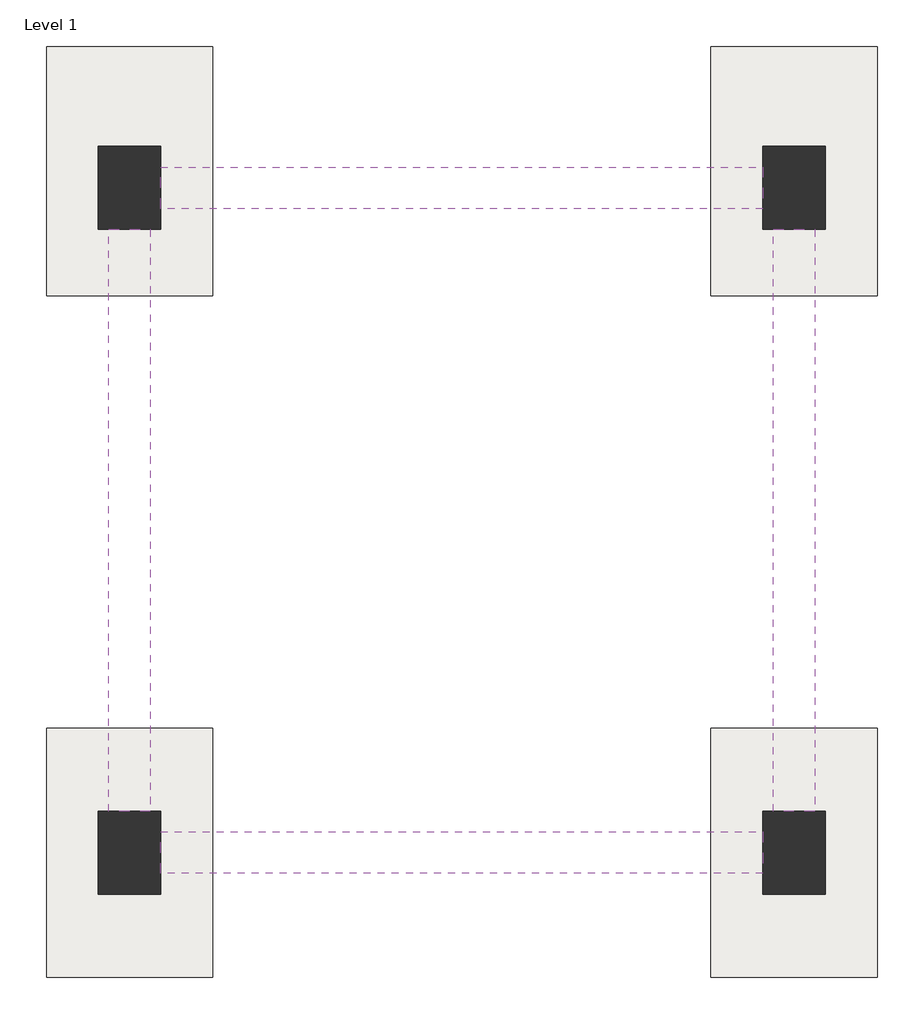
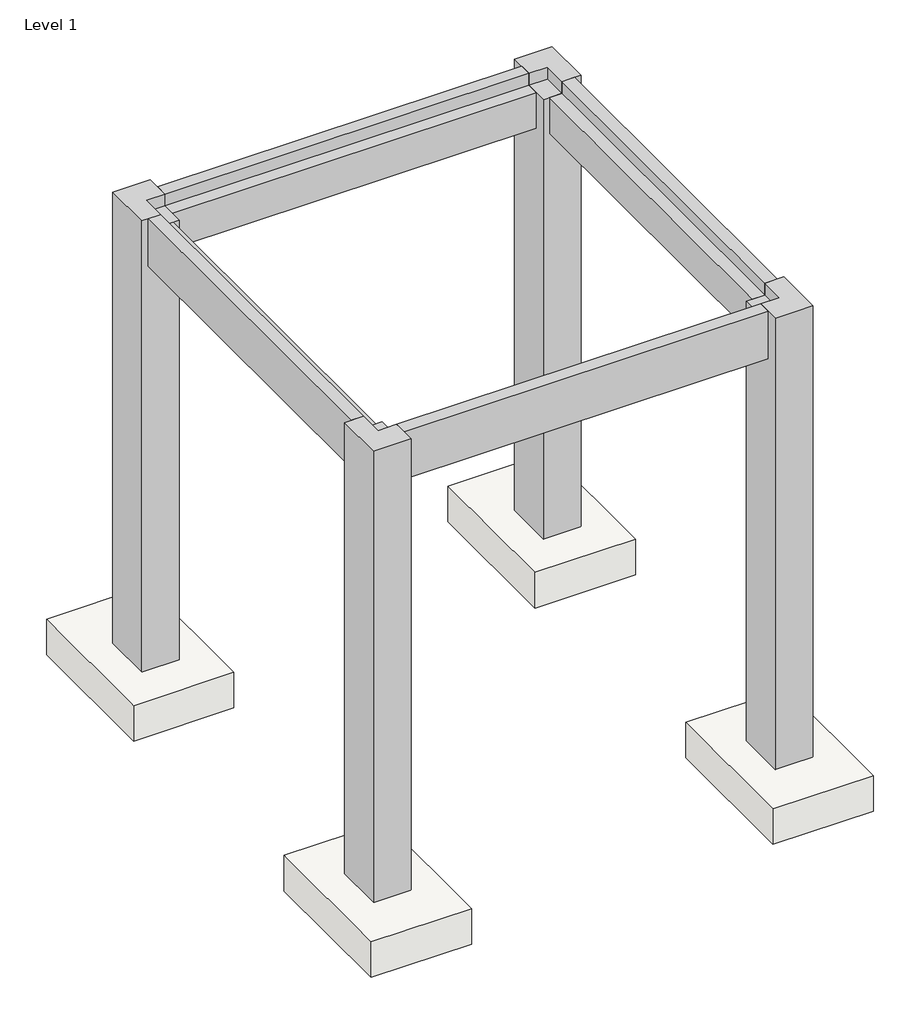
# One storey: 4 beams, 4 columns, 4 slabs.
"""IFC4 building model written with IfcOpenShell, lengths in millimetres."""

import ifcopenshell
import ifcopenshell.guid

model = None  # the IFC model being written
_history = None  # IfcOwnerHistory: only IFC2X3 demands one
_inside = {}  # id of a spatial element -> (the spatial element, [elements in it])
_under = {}  # id of a project, library or spatial element -> (it, [spatial elements below it])
_declared = {}  # id of a project -> (the project, [libraries it declares])
_typed = {}  # id of a type object -> (the type object, [elements of that type])
_made_of = {}  # id of a material, layer set ... -> (it, [elements and type objects made of it])


def new_model(schema):
    """Start an empty IFC model of exactly this schema.

    Asked for "IFC4X3", IfcOpenShell would pick the latest addendum, in which some entities
    have other attributes; the version numbers below select the first issue.
    IFC2X3 requires an IfcOwnerHistory on every rooted entity: one is made here for all.
    """
    global model, _history
    if schema == "IFC4X3":
        model = ifcopenshell.file(schema_version=(4, 3, 0, 0))
    else:
        model = ifcopenshell.file(schema=schema)
    _inside.clear()
    _under.clear()
    _declared.clear()
    _typed.clear()
    _made_of.clear()
    _history = None
    if model.schema == "IFC2X3":
        org = make("IfcOrganization", Name="unknown")
        user = make(
            "IfcPersonAndOrganization",
            ThePerson=make("IfcPerson", FamilyName="unknown"),
            TheOrganization=org,
        )
        app = make(
            "IfcApplication",
            ApplicationDeveloper=org,
            Version="unknown",
            ApplicationFullName="unknown",
            ApplicationIdentifier="unknown",
        )
        _history = make(
            "IfcOwnerHistory",
            OwningUser=user,
            OwningApplication=app,
            ChangeAction="ADDED",
            CreationDate=0,
        )
    return model


def make(cls, **values):
    """One entity of the class cls with the attributes given. An attribute that is None is left unset."""
    return model.create_entity(
        cls, **{name: value for name, value in values.items() if value is not None}
    )


def rooted(cls, **values):
    """An entity with a GlobalId (a new one), such as an element, a storey or a relation."""
    return make(cls, GlobalId=ifcopenshell.guid.new(), OwnerHistory=_history, **values)


def si_unit(unit_type, name, prefix=None):
    """IfcSIUnit, for example si_unit("LENGTHUNIT", "METRE", prefix="MILLI")."""
    return make("IfcSIUnit", UnitType=unit_type, Prefix=prefix, Name=name)


def assignment(units):
    """IfcUnitAssignment: the units of a project."""
    return None if units is None else make("IfcUnitAssignment", Units=units)


def point(xyz):
    """IfcCartesianPoint."""
    return None if xyz is None else make("IfcCartesianPoint", Coordinates=xyz)


def direction(xyz):
    """IfcDirection."""
    return None if xyz is None else make("IfcDirection", DirectionRatios=xyz)


def frame(location, z_axis=None, x_axis=None):
    """IfcAxis2Placement3D, a coordinate frame: its origin and axes. An axis left out is left unset."""
    return make(
        "IfcAxis2Placement3D",
        Location=point(location),
        Axis=direction(z_axis),
        RefDirection=direction(x_axis),
    )


def origin():
    """The frame at (0, 0, 0) with its axes left unset."""
    return frame((0.0, 0.0, 0.0))


def place(relative_to, where):
    """IfcLocalPlacement: puts the frame where relative to a parent placement (None: the world)."""
    return make(
        "IfcLocalPlacement", PlacementRelTo=relative_to, RelativePlacement=where
    )


def context(
    kind, dimensions, precision=None, world=None, true_north=None, identifier=None
):
    """IfcGeometricRepresentationContext, for example the 3D "Model" context."""
    return make(
        "IfcGeometricRepresentationContext",
        ContextIdentifier=identifier,
        ContextType=kind,
        CoordinateSpaceDimension=dimensions,
        Precision=precision,
        WorldCoordinateSystem=world,
        TrueNorth=true_north,
    )


def project(units=None, contexts=None):
    """IfcProject with its units and contexts."""
    return rooted(
        "IfcProject",
        Name="project",
        RepresentationContexts=contexts,
        UnitsInContext=assignment(units),
    )


def spatial(cls, under=None, at=None, **own):
    """A site, building, storey or space (cls), placed at a placement, below another one or the project."""
    s = rooted(cls, ObjectPlacement=at, **own)
    if under is not None:
        _under.setdefault(under.id(), (under, []))[1].append(s)
    return s


def polyline(points):
    """IfcPolyline through the points."""
    return make("IfcPolyline", Points=[point(p) for p in points])


def outline(outer, holes=None, kind="AREA"):
    """IfcArbitraryClosedProfileDef: a profile drawn as a closed curve; with holes, ...WithVoids."""
    if holes is None:
        return make("IfcArbitraryClosedProfileDef", ProfileType=kind, OuterCurve=outer)
    return make(
        "IfcArbitraryProfileDefWithVoids",
        ProfileType=kind,
        OuterCurve=outer,
        InnerCurves=holes,
    )


def extrude(swept, where, along, depth):
    """IfcExtrudedAreaSolid: the profile swept, set in the frame where, extruded along a direction by depth."""
    return make(
        "IfcExtrudedAreaSolid",
        SweptArea=swept,
        Position=where,
        ExtrudedDirection=direction(along),
        Depth=depth,
    )


def faces_of(points, faces, orient=None, outer=None):
    """IfcFace entities. A face is a list of loops; a loop is a list of indices into points, from 0.

    orient and outer hold one flag for each loop. By default every Orientation is true, the
    first loop of a face is its IfcFaceOuterBound and the others are IfcFaceBound.
    """
    made = []
    for i, loops in enumerate(faces):
        bounds = []
        for j, loop in enumerate(loops):
            is_outer = j == 0 if outer is None else outer[i][j]
            bounds.append(
                make(
                    "IfcFaceOuterBound" if is_outer else "IfcFaceBound",
                    Bound=make("IfcPolyLoop", Polygon=[points[k] for k in loop]),
                    Orientation=True if orient is None else orient[i][j],
                )
            )
        made.append(make("IfcFace", Bounds=bounds))
    return made


def faceted_brep(points, faces, orient=None, outer=None, voids=None):
    """IfcFacetedBrep: a solid bounded by flat faces; with voids (closed shells), ...WithVoids."""
    shared = [point(p) for p in points]
    hull = make("IfcClosedShell", CfsFaces=faces_of(shared, faces, orient, outer))
    if voids is None:
        return make("IfcFacetedBrep", Outer=hull)
    return make(
        "IfcFacetedBrepWithVoids",
        Outer=hull,
        Voids=[
            make(cls, CfsFaces=faces_of(shared, fs, o, b)) for cls, fs, o, b in voids
        ],
    )


def shape(context_of_items, identifier, shape_type, items):
    """IfcShapeRepresentation: the items that make up one representation, for example the "Body"."""
    return make(
        "IfcShapeRepresentation",
        ContextOfItems=context_of_items,
        RepresentationIdentifier=identifier,
        RepresentationType=shape_type,
        Items=items,
    )


def source(mapping_origin, context_of_items, identifier, shape_type, items):
    """IfcRepresentationMap: a shape defined once, which mapped items show again and again."""
    return make(
        "IfcRepresentationMap",
        MappingOrigin=mapping_origin,
        MappedRepresentation=shape(context_of_items, identifier, shape_type, items),
    )


def transform(
    local_origin,
    x_axis=None,
    y_axis=None,
    z_axis=None,
    scale=None,
    scale2=None,
    scale3=None,
    uniform=True,
):
    """IfcCartesianTransformationOperator3D, or its non-uniform kind. x_axis, y_axis, z_axis: its Axis1, 2, 3."""
    if uniform:
        return make(
            "IfcCartesianTransformationOperator3D",
            Axis1=direction(x_axis),
            Axis2=direction(y_axis),
            LocalOrigin=point(local_origin),
            Scale=scale,
            Axis3=direction(z_axis),
        )
    return make(
        "IfcCartesianTransformationOperator3DnonUniform",
        Axis1=direction(x_axis),
        Axis2=direction(y_axis),
        LocalOrigin=point(local_origin),
        Scale=scale,
        Axis3=direction(z_axis),
        Scale2=scale2,
        Scale3=scale3,
    )


def mapped(mapping_source, mapping_target):
    """IfcMappedItem: shows the shape of a source again, moved by a transform."""
    return make(
        "IfcMappedItem", MappingSource=mapping_source, MappingTarget=mapping_target
    )


def made_of(thing, what):
    """Note that an element or type object is made of a material, layer set ...; save() writes the relation."""
    if what is not None:
        _made_of.setdefault(what.id(), (what, []))[1].append(thing)
    return thing


def element(
    cls,
    number,
    at=None,
    inside=None,
    cuts=None,
    type_object=None,
    material=None,
    context=None,
    identifier="Body",
    shape_type=None,
    held_by="IfcProductDefinitionShape",
    body=None,
    shapes=None,
    **own,
):
    """One element of the class cls, such as IfcWall. Its Tag is "e" and its number.

    at: its placement. inside: the storey or other place that contains it. cuts: it is an
    opening in that element (IfcRelVoidsElement). A single representation is given by context,
    identifier, shape_type and body (its items); several are given by shapes. held_by: the class
    of the entity that holds the representations. save() writes the other relations.
    """
    e = rooted(cls, Tag="e%d" % number, ObjectPlacement=at, **own)
    if body is not None:
        shapes = [shape(context, identifier, shape_type, body)]
    if shapes is not None:
        e.Representation = make(held_by, Representations=shapes)
    if inside is not None:
        _inside.setdefault(inside.id(), (inside, []))[1].append(e)
    if cuts is not None:
        rooted(
            "IfcRelVoidsElement", RelatingBuildingElement=cuts, RelatedOpeningElement=e
        )
    if type_object is not None:
        _typed.setdefault(type_object.id(), (type_object, []))[1].append(e)
    return made_of(e, material)


def aggregate(whole, parts):
    """IfcRelAggregates: a whole, such as a stair, and the parts it consists of."""
    return rooted("IfcRelAggregates", RelatingObject=whole, RelatedObjects=parts)


def save(model, path):
    """Write the relations noted so far, then the file.

    IfcRelAggregates (storeys below a building ...), IfcRelContainedInSpatialStructure (elements
    in a storey), IfcRelDefinesByType, IfcRelAssociatesMaterial and IfcRelDeclares: one each for
    every whole, place, type object, material and project.
    """
    for whole, parts in _under.values():
        aggregate(whole, parts)
    for where, things in _inside.values():
        rooted(
            "IfcRelContainedInSpatialStructure",
            RelatedElements=things,
            RelatingStructure=where,
        )
    for kind, things in _typed.values():
        rooted("IfcRelDefinesByType", RelatedObjects=things, RelatingType=kind)
    for what, things in _made_of.values():
        rooted("IfcRelAssociatesMaterial", RelatedObjects=things, RelatingMaterial=what)
    for by, libraries in _declared.values():
        rooted("IfcRelDeclares", RelatingContext=by, RelatedDefinitions=libraries)
    model.write(path)


def slab_5ba74754(model_context):
    return source(origin(), model_context, "Body", "SweptSolid", [
        extrude(outline(polyline([(609.6, 914.4), (609.6, -914.4), (-609.6, -914.4), (-609.6, 914.4), (609.6, 914.4)])), frame((0.0, 0.0, -457.2), z_axis=(0.0, 0.0, 1.0), x_axis=(1.0, 0.0, 0.0)), (0.0, 0.0, 1.0), 457.2),
    ])


model = new_model("IFC4")

# Units and contexts
model_context = context("Model", 3, world=origin())
ifc_project = project(units=[si_unit("LENGTHUNIT", "METRE", prefix="MILLI")], contexts=[model_context])

# Site, building, storey
site = spatial("IfcSite", under=ifc_project)
building = spatial("IfcBuilding", under=site)
storey = spatial("IfcBuildingStorey", under=building, Name="Level 1", Elevation=0.0)

# Beams
placement = place(None, origin())
element("IfcBeam", 1, ObjectType="Concrete-Rectangular Beam : 12 x 24", at=placement, inside=storey, context=model_context, shape_type="SweptSolid", body=[
    extrude(outline(polyline([(786.0323826, 2438.4), (786.0323826, 3048.0), (938.4323826, 3048.0), (938.4323826, 2895.6), (1090.8323826, 2895.6), (1090.8323826, 2438.4), (786.0323826, 2438.4)])), frame((-11045.0800525, 0.0, 0.0), z_axis=(1.0, 0.0, 0.0), x_axis=(0.0, 1.0, 0.0)), (0.0, 0.0, 1.0), 4419.6),
])
element("IfcBeam", 2, ObjectType="Concrete-Rectangular Beam : 12 x 24", at=placement, inside=storey, context=model_context, shape_type="SweptSolid", body=[
    extrude(outline(polyline([(5967.6323826, 3048.0), (5967.6323826, 2438.4), (5662.8323826, 2438.4), (5662.8323826, 2895.6), (5815.2323826, 2895.6), (5815.2323826, 3048.0), (5967.6323826, 3048.0)])), frame((-11045.0800525, 0.0, 0.0), z_axis=(1.0, 0.0, 0.0), x_axis=(0.0, 1.0, 0.0)), (0.0, 0.0, 1.0), 4419.6),
])
element("IfcBeam", 3, ObjectType="Concrete-Rectangular Beam : 12 x 24", at=placement, inside=storey, context=model_context, shape_type="SweptSolid", body=[
    extrude(outline(polyline([(2438.4, -11426.0800525), (2438.4, -11121.2800525), (2895.6, -11121.2800525), (2895.6, -11273.6800525), (3048.0, -11273.6800525), (3048.0, -11426.0800525), (2438.4, -11426.0800525)])), frame((0.0, 1243.2323826, 0.0), z_axis=(0.0, 1.0, 0.0), x_axis=(0.0, 0.0, 1.0)), (0.0, 0.0, 1.0), 4267.2),
])
element("IfcBeam", 4, ObjectType="Concrete-Rectangular Beam : 12 x 24", at=placement, inside=storey, context=model_context, shape_type="SweptSolid", body=[
    extrude(outline(polyline([(2438.4, -6244.4800525), (3048.0, -6244.4800525), (3048.0, -6396.8800525), (2895.6, -6396.8800525), (2895.6, -6549.2800525), (2438.4, -6549.2800525), (2438.4, -6244.4800525)])), frame((0.0, 1243.2323826, 0.0), z_axis=(0.0, 1.0, 0.0), x_axis=(0.0, 0.0, 1.0)), (0.0, 0.0, 1.0), 4267.2),
])

# Columns
element("IfcColumn", 5, ObjectType="Concrete-Rectangular-Column : 18 x 24", at=placement, inside=storey, context=model_context, shape_type="Brep", body=[
    faceted_brep([(-11045.0800525, 6120.0323826, 3048.0), (-11502.2800525, 6120.0323826, 3048.0), (-11502.2800525, 5510.4323826, 3048.0), (-11273.6800525, 5510.4323826, 3048.0), (-11273.6800525, 5815.2323826, 3048.0), (-11045.0800525, 5815.2323826, 3048.0), (-11045.0800525, 6120.0323826, -2743.2), (-11045.0800525, 5510.4323826, -2743.2), (-11502.2800525, 5510.4323826, -2743.2), (-11502.2800525, 6120.0323826, -2743.2), (-11045.0800525, 5510.4323826, 2895.6), (-11273.6800525, 5510.4323826, 2895.6), (-11045.0800525, 5815.2323826, 2895.6), (-11273.6800525, 5815.2323826, 2895.6)], [[[0, 1, 2, 3, 4, 5]], [[6, 7, 8, 9]], [[1, 0, 6, 9]], [[2, 1, 9, 8]], [[8, 7, 10, 11, 3, 2]], [[7, 6, 0, 5, 12, 10]], [[13, 11, 10, 12]], [[4, 13, 12, 5]], [[13, 4, 3, 11]]]),
])
element("IfcColumn", 6, ObjectType="Concrete-Rectangular-Column : 18 x 24", at=placement, inside=storey, context=model_context, shape_type="Brep", body=[
    faceted_brep([(-6168.2800525, 6120.0323826, 3048.0), (-6625.4800525, 6120.0323826, 3048.0), (-6625.4800525, 5815.2323826, 3048.0), (-6396.8800525, 5815.2323826, 3048.0), (-6396.8800525, 5510.4323826, 3048.0), (-6168.2800525, 5510.4323826, 3048.0), (-6168.2800525, 6120.0323826, -2743.2), (-6168.2800525, 5510.4323826, -2743.2), (-6625.4800525, 5510.4323826, -2743.2), (-6625.4800525, 6120.0323826, -2743.2), (-6625.4800525, 5510.4323826, 2895.6), (-6625.4800525, 5815.2323826, 2895.6), (-6396.8800525, 5510.4323826, 2895.6), (-6396.8800525, 5815.2323826, 2895.6)], [[[0, 1, 2, 3, 4, 5]], [[6, 7, 8, 9]], [[1, 0, 6, 9]], [[9, 8, 10, 11, 2, 1]], [[8, 7, 5, 4, 12, 10]], [[0, 5, 7, 6]], [[12, 13, 11, 10]], [[13, 3, 2, 11]], [[3, 13, 12, 4]]]),
])
element("IfcColumn", 7, ObjectType="Concrete-Rectangular-Column : 18 x 24", at=placement, inside=storey, context=model_context, shape_type="Brep", body=[
    faceted_brep([(-11502.2800525, 1243.2323826, 3048.0), (-11502.2800525, 633.6323826, 3048.0), (-11045.0800525, 633.6323826, 3048.0), (-11045.0800525, 938.4323826, 3048.0), (-11273.6800525, 938.4323826, 3048.0), (-11273.6800525, 1243.2323826, 3048.0), (-11045.0800525, 1243.2323826, -2743.2), (-11045.0800525, 633.6323826, -2743.2), (-11502.2800525, 633.6323826, -2743.2), (-11502.2800525, 1243.2323826, -2743.2), (-11273.6800525, 1243.2323826, 2895.6), (-11045.0800525, 1243.2323826, 2895.6), (-11045.0800525, 938.4323826, 2895.6), (-11273.6800525, 938.4323826, 2895.6)], [[[0, 1, 2, 3, 4, 5]], [[6, 7, 8, 9]], [[6, 9, 0, 5, 10, 11]], [[1, 0, 9, 8]], [[2, 1, 8, 7]], [[7, 6, 11, 12, 3, 2]], [[10, 13, 12, 11]], [[13, 4, 3, 12]], [[4, 13, 10, 5]]]),
])
element("IfcColumn", 8, ObjectType="Concrete-Rectangular-Column : 18 x 24", at=placement, inside=storey, context=model_context, shape_type="Brep", body=[
    faceted_brep([(-6625.4800525, 633.6323826, 3048.0), (-6168.2800525, 633.6323826, 3048.0), (-6168.2800525, 1243.2323826, 3048.0), (-6396.8800525, 1243.2323826, 3048.0), (-6396.8800525, 938.4323826, 3048.0), (-6625.4800525, 938.4323826, 3048.0), (-6168.2800525, 1243.2323826, -2743.2), (-6168.2800525, 633.6323826, -2743.2), (-6625.4800525, 633.6323826, -2743.2), (-6625.4800525, 1243.2323826, -2743.2), (-6625.4800525, 1243.2323826, 2895.6), (-6396.8800525, 1243.2323826, 2895.6), (-6625.4800525, 938.4323826, 2895.6), (-6396.8800525, 938.4323826, 2895.6)], [[[0, 1, 2, 3, 4, 5]], [[6, 7, 8, 9]], [[6, 9, 10, 11, 3, 2]], [[9, 8, 0, 5, 12, 10]], [[1, 0, 8, 7]], [[2, 1, 7, 6]], [[12, 13, 11, 10]], [[13, 4, 3, 11]], [[4, 13, 12, 5]]]),
])

# Slabs
slab_shape = slab_5ba74754(model_context)
element("IfcSlab", 9, ObjectType="Footing-Rectangular : 72\" x 48\" x 18\"", at=placement, inside=storey, context=model_context, shape_type="MappedRepresentation", body=[
    mapped(slab_shape, transform((-11273.6800525, 5938.4323826, -2743.2), x_axis=(1.0, 0.0, 0.0), y_axis=(0.0, 1.0, 0.0), z_axis=(0.0, 0.0, 1.0))),
])
element("IfcSlab", 10, ObjectType="Footing-Rectangular : 72\" x 48\" x 18\"", at=placement, inside=storey, context=model_context, shape_type="MappedRepresentation", body=[
    mapped(slab_shape, transform((-6396.8800525, 5938.4323826, -2743.2), x_axis=(1.0, 0.0, 0.0), y_axis=(0.0, 1.0, 0.0), z_axis=(0.0, 0.0, 1.0))),
])
element("IfcSlab", 11, ObjectType="Footing-Rectangular : 72\" x 48\" x 18\"", at=placement, inside=storey, context=model_context, shape_type="MappedRepresentation", body=[
    mapped(slab_shape, transform((-11273.6800525, 938.4323826, -2743.2), x_axis=(1.0, 0.0, 0.0), y_axis=(0.0, 1.0, 0.0), z_axis=(0.0, 0.0, 1.0))),
])
element("IfcSlab", 12, ObjectType="Footing-Rectangular : 72\" x 48\" x 18\"", at=placement, inside=storey, context=model_context, shape_type="MappedRepresentation", body=[
    mapped(slab_shape, transform((-6396.8800525, 938.4323826, -2743.2), x_axis=(1.0, 0.0, 0.0), y_axis=(0.0, 1.0, 0.0), z_axis=(0.0, 0.0, 1.0))),
])

save(model, "model.ifc")

# Revit data of these elements
# Project information
#   Project Issue Date = "Issue Date"
#   Project Status = "Project Status"
#   Client Name = "Owner"
#   Project Address = "Enter address here"
#   Project Name = "Project Name"
#   Project Number = "Project Number"
# Grids (mm)
#   "1": line (9019.216, 5815.232) -> (-21563.036, 5815.232)
#   "2": line (-11273.68, -9686.145) -> (-11273.68, 17085.235)
#   "3": line (-6396.88, 17085.235) -> (-6396.88, -9686.145)
#   "4.78": line (9019.216, 938.432) -> (-21563.036, 938.432)
# Type "Concrete-Rectangular Beam : 12 x 24"
#   Assembly Code = "B10"
#   Length [instance default] = 1.524 m
#   b = 0.3048 m
#   h = 0.6096 m
#   Structural Material [instance default] = Concrete - Cast-in-Place Concrete
# Type "Concrete-Rectangular-Column : 18 x 24"
#   Assembly Code = "B10"
#   b = 0.4572 m
#   h = 0.6096 m
#   Structural Material [instance default] = Concrete - Cast-in-Place Concrete
# Type "Footing-Rectangular : 72\" x 48\" x 18\""
#   Assembly Code = "A1010100"
#   Width = 1.2192 m
#   Length = 1.8288 m
#   Thickness = 0.4572 m
#   Structural Material [instance default] = Concrete - Cast-in-Place Concrete
# Elements 1, 2, 3, 4 (IfcBeam, "Concrete-Rectangular Beam : 12 x 24")
#   Comments = ""
#   Structural Material = Concrete - Cast-in-Place Concrete
#   Phase Created = New Construction
#   Materials on its faces: "Concrete - Cast-in-Place Concrete"
# Elements 5, 6, 7, 8 (IfcColumn, "Concrete-Rectangular-Column : 18 x 24")
#   Structural Material = Concrete - Cast-in-Place Concrete
#   Phase Created = New Construction
#   Materials on its faces: "Concrete - Cast-in-Place Concrete"
# Element 9 (IfcSlab, "Footing-Rectangular : 72\" x 48\" x 18\"")
#   Structural Material = Concrete - Cast-in-Place Concrete
#   Phase Created = New Construction
#   Materials on its faces: "Concrete - Cast-in-Place Concrete"
# Elements 10, 11, 12 (IfcSlab, "Footing-Rectangular : 72\" x 48\" x 18\"")
#   Comments = ""
#   Structural Material = Concrete - Cast-in-Place Concrete
#   Phase Created = New Construction
#   Materials on its faces: "Concrete - Cast-in-Place Concrete"
# Materials
#   "Concrete - Cast-in-Place Concrete": class "Concrete", colour RGB 192 192 192, transparency 0
